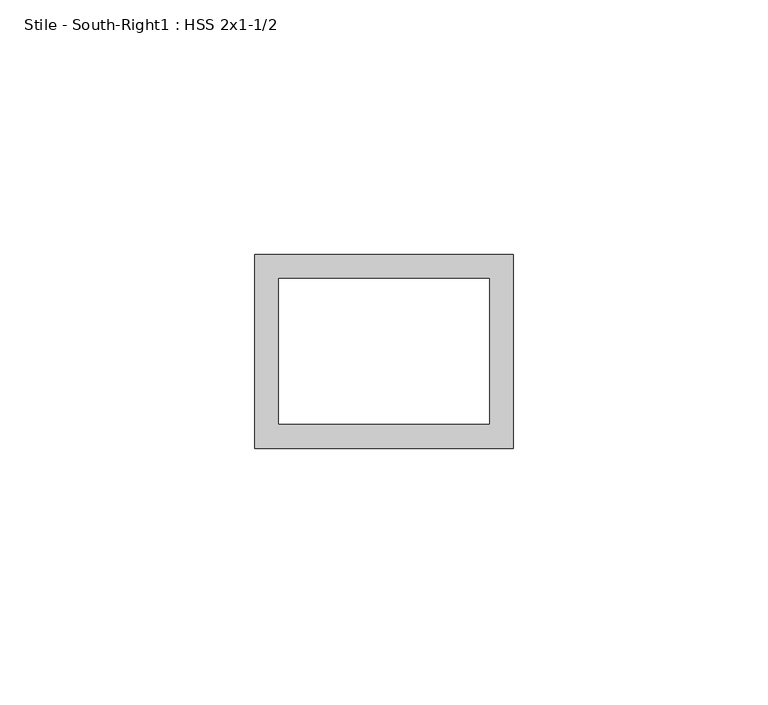
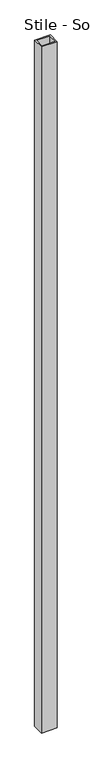
"""IFC4 building model written with IfcOpenShell, lengths in millimetres: proxy geometry, Stile - South-Right1 : HSS 2x1-1/2."""

from ifc_helpers import new_model, si_unit, frame, origin, place, context, project, spatial, polyline, outline, extrude, source, transform, mapped, element, save


def stile_south_right1_hss_2x1_1_2_42ef625e(model_context):
    return source(origin(), model_context, "Body", "SweptSolid", [
        extrude(outline(polyline([(587365.8934739, -536263.6038841), (587416.6934739, -536263.6038841), (587416.6934739, -536301.7038841), (587365.8934739, -536301.7038841), (587365.8934739, -536263.6038841)]), holes=[polyline([(587370.6559739, -536268.3663841), (587370.6559739, -536296.9413841), (587411.9309739, -536296.9413841), (587411.9309739, -536268.3663841), (587370.6559739, -536268.3663841)])]), frame((0.0, 0.0, 50.8), z_axis=(0.0, 0.0, 1.0), x_axis=(1.0, 0.0, 0.0)), (0.0, 0.0, 1.0), 2349.5),
    ])


if __name__ == "__main__":
    model = new_model("IFC4")
    model_context = context("Model", 3, world=origin())
    ifc_project = project(units=[si_unit("LENGTHUNIT", "METRE", prefix="MILLI")], contexts=[model_context])
    site = spatial("IfcSite", under=ifc_project)
    building = spatial("IfcBuilding", under=site)
    placement = place(None, origin())
    stile_south_right1_hss_2x1_1_2_shape = stile_south_right1_hss_2x1_1_2_42ef625e(model_context)
    element("IfcBuildingElementProxy", 1, Name="Stile - South-Right1 : HSS 2x1-1/2", ObjectType="Stile - South-Right1 : HSS 2x1-1/2", at=placement, inside=building, context=model_context, shape_type="MappedRepresentation", body=[
        mapped(stile_south_right1_hss_2x1_1_2_shape, transform((0.0, 0.0, 0.0), x_axis=(1.0, 0.0, 0.0), y_axis=(0.0, 1.0, 0.0), z_axis=(0.0, 0.0, 1.0))),
    ])
    save(model, "model.ifc")

# Revit data of these elements
# Element 1 (IfcBuildingElementProxy, "Stile - South-Right1 : HSS 2x1-1/2")
#   Materials on its faces: "1-1/2\"X2\" GALV. STL HSS TUBING"
# Materials
#   "1-1/2\"X2\" GALV. STL HSS TUBING": class "Generic", colour RGB 211 211 207, transparency 0, Cost = 0
